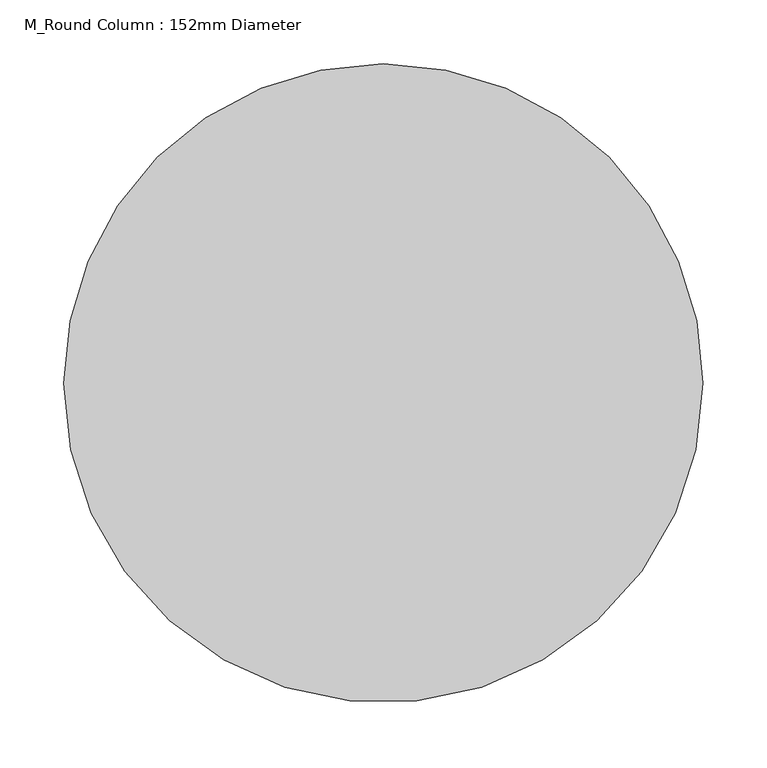
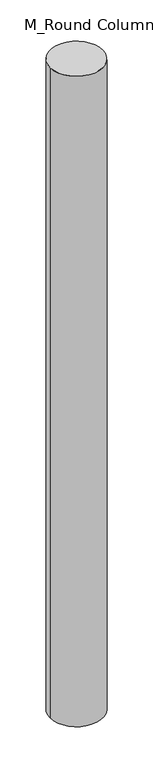
"""IFC4 building model written with IfcOpenShell, lengths in millimetres: column geometry, M_Round Column : 152mm Diameter."""

from ifc_helpers import new_model, si_unit, point, frame, origin, origin_2d, place, context, project, spatial, circle_curve, trimmed, segment, composite_curve, outline, extrude, source, transform, mapped, element, save


def m_round_column_152mm_diameter_4ccac3bb(model_context):
    return source(origin(), model_context, "Body", "SweptSolid", [
        extrude(outline(composite_curve([segment(trimmed(circle_curve(origin_2d(), 250.0), [point((250.0, 0.0))], [point((-250.0, 0.0))], False, "CARTESIAN"), True, "CONTINUOUS"), segment(trimmed(circle_curve(origin_2d(), 250.0), [point((-250.0, 0.0))], [point((0.0, 250.0))], False, "CARTESIAN"), True, "CONTINUOUS"), segment(trimmed(circle_curve(origin_2d(), 250.0), [point((0.0, 250.0))], [point((250.0, 0.0))], False, "CARTESIAN"), True, "CONTINUOUS")], self_intersect=False)), frame((0.0, 0.0, 11500.0), z_axis=(0.0, 0.0, 1.0), x_axis=(1.0, 0.0, 0.0)), (0.0, 0.0, 1.0), 6500.0),
    ])


if __name__ == "__main__":
    model = new_model("IFC4")
    model_context = context("Model", 3, world=origin())
    ifc_project = project(units=[si_unit("LENGTHUNIT", "METRE", prefix="MILLI")], contexts=[model_context])
    site = spatial("IfcSite", under=ifc_project)
    building = spatial("IfcBuilding", under=site)
    placement = place(None, origin())
    m_round_column_152mm_diameter_shape = m_round_column_152mm_diameter_4ccac3bb(model_context)
    element("IfcColumn", 1, ObjectType="M_Round Column : 152mm Diameter", at=placement, inside=building, context=model_context, shape_type="MappedRepresentation", body=[
        mapped(m_round_column_152mm_diameter_shape, transform((0.0, 0.0, 0.0), x_axis=(1.0, 0.0, 0.0), y_axis=(0.0, 1.0, 0.0), z_axis=(0.0, 0.0, 1.0))),
    ])
    save(model, "model.ifc")

# Revit data of these elements
# Type "M_Round Column : 152mm Diameter"
#   Diameter = 0.5 m
#   Offset Base = 0 m
#   Offset Top = 0 m
#   Material = none
